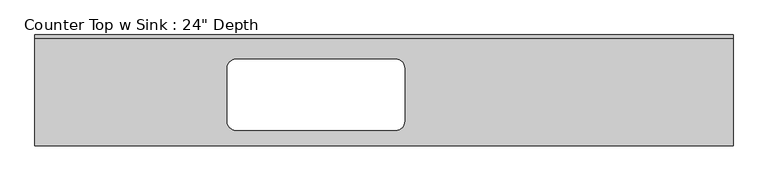
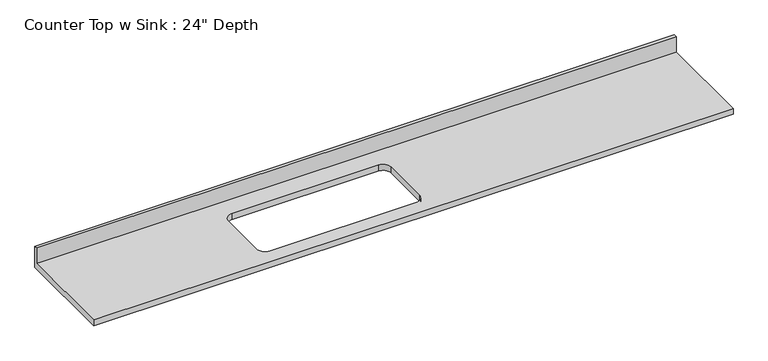
"""IFC4 building model written with IfcOpenShell, lengths in millimetres: furniture geometry."""

import ifcopenshell
import ifcopenshell.guid

model = None  # the IFC model being written
_history = None  # IfcOwnerHistory: only IFC2X3 demands one
_inside = {}  # id of a spatial element -> (the spatial element, [elements in it])
_under = {}  # id of a project, library or spatial element -> (it, [spatial elements below it])
_declared = {}  # id of a project -> (the project, [libraries it declares])
_typed = {}  # id of a type object -> (the type object, [elements of that type])
_made_of = {}  # id of a material, layer set ... -> (it, [elements and type objects made of it])


def new_model(schema):
    """Start an empty IFC model of exactly this schema.

    Asked for "IFC4X3", IfcOpenShell would pick the latest addendum, in which some entities
    have other attributes; the version numbers below select the first issue.
    IFC2X3 requires an IfcOwnerHistory on every rooted entity: one is made here for all.
    """
    global model, _history
    if schema == "IFC4X3":
        model = ifcopenshell.file(schema_version=(4, 3, 0, 0))
    else:
        model = ifcopenshell.file(schema=schema)
    _inside.clear()
    _under.clear()
    _declared.clear()
    _typed.clear()
    _made_of.clear()
    _history = None
    if model.schema == "IFC2X3":
        org = make("IfcOrganization", Name="unknown")
        user = make(
            "IfcPersonAndOrganization",
            ThePerson=make("IfcPerson", FamilyName="unknown"),
            TheOrganization=org,
        )
        app = make(
            "IfcApplication",
            ApplicationDeveloper=org,
            Version="unknown",
            ApplicationFullName="unknown",
            ApplicationIdentifier="unknown",
        )
        _history = make(
            "IfcOwnerHistory",
            OwningUser=user,
            OwningApplication=app,
            ChangeAction="ADDED",
            CreationDate=0,
        )
    return model


def make(cls, **values):
    """One entity of the class cls with the attributes given. An attribute that is None is left unset."""
    return model.create_entity(
        cls, **{name: value for name, value in values.items() if value is not None}
    )


def rooted(cls, **values):
    """An entity with a GlobalId (a new one), such as an element, a storey or a relation."""
    return make(cls, GlobalId=ifcopenshell.guid.new(), OwnerHistory=_history, **values)


def si_unit(unit_type, name, prefix=None):
    """IfcSIUnit, for example si_unit("LENGTHUNIT", "METRE", prefix="MILLI")."""
    return make("IfcSIUnit", UnitType=unit_type, Prefix=prefix, Name=name)


def assignment(units):
    """IfcUnitAssignment: the units of a project."""
    return None if units is None else make("IfcUnitAssignment", Units=units)


def point(xyz):
    """IfcCartesianPoint."""
    return None if xyz is None else make("IfcCartesianPoint", Coordinates=xyz)


def direction(xyz):
    """IfcDirection."""
    return None if xyz is None else make("IfcDirection", DirectionRatios=xyz)


def frame(location, z_axis=None, x_axis=None):
    """IfcAxis2Placement3D, a coordinate frame: its origin and axes. An axis left out is left unset."""
    return make(
        "IfcAxis2Placement3D",
        Location=point(location),
        Axis=direction(z_axis),
        RefDirection=direction(x_axis),
    )


def origin():
    """The frame at (0, 0, 0) with its axes left unset."""
    return frame((0.0, 0.0, 0.0))


def place(relative_to, where):
    """IfcLocalPlacement: puts the frame where relative to a parent placement (None: the world)."""
    return make(
        "IfcLocalPlacement", PlacementRelTo=relative_to, RelativePlacement=where
    )


def context(
    kind, dimensions, precision=None, world=None, true_north=None, identifier=None
):
    """IfcGeometricRepresentationContext, for example the 3D "Model" context."""
    return make(
        "IfcGeometricRepresentationContext",
        ContextIdentifier=identifier,
        ContextType=kind,
        CoordinateSpaceDimension=dimensions,
        Precision=precision,
        WorldCoordinateSystem=world,
        TrueNorth=true_north,
    )


def project(units=None, contexts=None):
    """IfcProject with its units and contexts."""
    return rooted(
        "IfcProject",
        Name="project",
        RepresentationContexts=contexts,
        UnitsInContext=assignment(units),
    )


def spatial(cls, under=None, at=None, **own):
    """A site, building, storey or space (cls), placed at a placement, below another one or the project."""
    s = rooted(cls, ObjectPlacement=at, **own)
    if under is not None:
        _under.setdefault(under.id(), (under, []))[1].append(s)
    return s


def polyline(points):
    """IfcPolyline through the points."""
    return make("IfcPolyline", Points=[point(p) for p in points])


def circle_curve(where, radius):
    """IfcCircle in the frame where."""
    return make("IfcCircle", Position=where, Radius=radius)


def shape(context_of_items, identifier, shape_type, items):
    """IfcShapeRepresentation: the items that make up one representation, for example the "Body"."""
    return make(
        "IfcShapeRepresentation",
        ContextOfItems=context_of_items,
        RepresentationIdentifier=identifier,
        RepresentationType=shape_type,
        Items=items,
    )


def source(mapping_origin, context_of_items, identifier, shape_type, items):
    """IfcRepresentationMap: a shape defined once, which mapped items show again and again."""
    return make(
        "IfcRepresentationMap",
        MappingOrigin=mapping_origin,
        MappedRepresentation=shape(context_of_items, identifier, shape_type, items),
    )


def transform(
    local_origin,
    x_axis=None,
    y_axis=None,
    z_axis=None,
    scale=None,
    scale2=None,
    scale3=None,
    uniform=True,
):
    """IfcCartesianTransformationOperator3D, or its non-uniform kind. x_axis, y_axis, z_axis: its Axis1, 2, 3."""
    if uniform:
        return make(
            "IfcCartesianTransformationOperator3D",
            Axis1=direction(x_axis),
            Axis2=direction(y_axis),
            LocalOrigin=point(local_origin),
            Scale=scale,
            Axis3=direction(z_axis),
        )
    return make(
        "IfcCartesianTransformationOperator3DnonUniform",
        Axis1=direction(x_axis),
        Axis2=direction(y_axis),
        LocalOrigin=point(local_origin),
        Scale=scale,
        Axis3=direction(z_axis),
        Scale2=scale2,
        Scale3=scale3,
    )


def mapped(mapping_source, mapping_target):
    """IfcMappedItem: shows the shape of a source again, moved by a transform."""
    return make(
        "IfcMappedItem", MappingSource=mapping_source, MappingTarget=mapping_target
    )


def made_of(thing, what):
    """Note that an element or type object is made of a material, layer set ...; save() writes the relation."""
    if what is not None:
        _made_of.setdefault(what.id(), (what, []))[1].append(thing)
    return thing


def element(
    cls,
    number,
    at=None,
    inside=None,
    cuts=None,
    type_object=None,
    material=None,
    context=None,
    identifier="Body",
    shape_type=None,
    held_by="IfcProductDefinitionShape",
    body=None,
    shapes=None,
    **own,
):
    """One element of the class cls, such as IfcWall. Its Tag is "e" and its number.

    at: its placement. inside: the storey or other place that contains it. cuts: it is an
    opening in that element (IfcRelVoidsElement). A single representation is given by context,
    identifier, shape_type and body (its items); several are given by shapes. held_by: the class
    of the entity that holds the representations. save() writes the other relations.
    """
    e = rooted(cls, Tag="e%d" % number, ObjectPlacement=at, **own)
    if body is not None:
        shapes = [shape(context, identifier, shape_type, body)]
    if shapes is not None:
        e.Representation = make(held_by, Representations=shapes)
    if inside is not None:
        _inside.setdefault(inside.id(), (inside, []))[1].append(e)
    if cuts is not None:
        rooted(
            "IfcRelVoidsElement", RelatingBuildingElement=cuts, RelatedOpeningElement=e
        )
    if type_object is not None:
        _typed.setdefault(type_object.id(), (type_object, []))[1].append(e)
    return made_of(e, material)


def aggregate(whole, parts):
    """IfcRelAggregates: a whole, such as a stair, and the parts it consists of."""
    return rooted("IfcRelAggregates", RelatingObject=whole, RelatedObjects=parts)


def save(model, path):
    """Write the relations noted so far, then the file.

    IfcRelAggregates (storeys below a building ...), IfcRelContainedInSpatialStructure (elements
    in a storey), IfcRelDefinesByType, IfcRelAssociatesMaterial and IfcRelDeclares: one each for
    every whole, place, type object, material and project.
    """
    for whole, parts in _under.values():
        aggregate(whole, parts)
    for where, things in _inside.values():
        rooted(
            "IfcRelContainedInSpatialStructure",
            RelatedElements=things,
            RelatingStructure=where,
        )
    for kind, things in _typed.values():
        rooted("IfcRelDefinesByType", RelatedObjects=things, RelatingType=kind)
    for what, things in _made_of.values():
        rooted("IfcRelAssociatesMaterial", RelatedObjects=things, RelatingMaterial=what)
    for by, libraries in _declared.values():
        rooted("IfcRelDeclares", RelatingContext=by, RelatedDefinitions=libraries)
    model.write(path)


def plane_surface(at):
    """IfcPlane: the flat surface through the origin of the frame at, square to its z axis."""
    return make("IfcPlane", Position=at)


def revolved_surface(curve, axis_point, axis_direction):
    """IfcSurfaceOfRevolution: the curve turned about the line through axis_point along axis_direction."""
    return make(
        "IfcSurfaceOfRevolution",
        SweptCurve=make("IfcArbitraryOpenProfileDef", ProfileType="CURVE", Curve=curve),
        AxisPosition=make("IfcAxis1Placement", Location=point(axis_point), Axis=direction(axis_direction)),
    )


def advanced_brep(points, edges, surfaces, faces):
    """IfcAdvancedBrep: a solid bounded by faces that lie on surfaces and meet in shared edges.

    An edge is (start, end): straight between two places in points (the first is 0);
    or (start, end, curve); or (start, end, curve, False) where it runs against its curve.
    A face is (place in surfaces, loops), or (place, loops, False) where it looks against
    its surface's normal. A loop lists edges by number (the first is 1), with a minus sign
    where the edge is run from its end to its start. The first loop is the outer one.
    """
    corners = [point(p) for p in points]
    vertices = [make("IfcVertexPoint", VertexGeometry=c) for c in corners]
    made = []
    for start, end, *more in edges:
        made.append(
            make(
                "IfcEdgeCurve",
                EdgeStart=vertices[start],
                EdgeEnd=vertices[end],
                EdgeGeometry=more[0] if more else make("IfcPolyline", Points=[corners[start], corners[end]]),
                SameSense=more[1] if len(more) > 1 else True,
            )
        )
    hull = []
    for where, loops, *sense in faces:
        bounds = []
        for j, loop in enumerate(loops):
            ring = [make("IfcOrientedEdge", EdgeElement=made[abs(k) - 1], Orientation=k > 0) for k in loop]
            bounds.append(
                make(
                    "IfcFaceOuterBound" if j == 0 else "IfcFaceBound",
                    Bound=make("IfcEdgeLoop", EdgeList=ring),
                    Orientation=True,
                )
            )
        hull.append(make("IfcAdvancedFace", Bounds=bounds, FaceSurface=surfaces[where], SameSense=sense[0] if sense else True))
    return make("IfcAdvancedBrep", Outer=make("IfcClosedShell", CfsFaces=hull))


def furniture_78cc09a6(model_context):
    return source(origin(), model_context, "Body", "AdvancedBrep", [
        advanced_brep(
        [(-1200.4622951, -635.0, 914.4), (2796.8627049, -635.0, 914.4), (2796.8627049, -19.05, 914.4), (-1200.4622951, -19.05, 914.4), (-48.9743878, -139.7, 914.4), (865.4256122, -139.7, 914.4), (916.2256122, -190.5, 914.4), (916.2256122, -495.3, 914.4), (865.4256122, -546.1, 914.4), (-48.9743878, -546.1, 914.4), (-99.7743878, -495.3, 914.4), (-99.7743878, -190.5, 914.4), (2796.8627049, 0.0, 876.3), (2796.8627049, -635.0, 876.3), (-1200.4622951, -635.0, 876.3), (-1200.4622951, 0.0, 876.3), (865.4256122, -139.7, 876.3), (-48.9743878, -139.7, 876.3), (-99.7743878, -190.5, 876.3), (-99.7743878, -495.3, 876.3), (-48.9743878, -546.1, 876.3), (865.4256122, -546.1, 876.3), (916.2256122, -495.3, 876.3), (916.2256122, -190.5, 876.3), (-1200.4622951, 0.0, 1016.0), (2796.8627049, 0.0, 1016.0), (-1200.4622951, -19.05, 1016.0), (2796.8627049, -19.05, 1016.0)],
        [
            (0, 1),
            (1, 2),
            (2, 3),
            (3, 0),
            (4, 5),
            (5, 6, circle_curve(frame((865.4256122, -190.5, 914.4), z_axis=(0.0, 0.0, -1.0), x_axis=(1.0, 0.0, 0.0)), 50.8)),
            (6, 7),
            (7, 8, circle_curve(frame((865.4256122, -495.3, 914.4), z_axis=(0.0, 0.0, -1.0), x_axis=(1.0, 0.0, 0.0)), 50.8)),
            (8, 9),
            (9, 10, circle_curve(frame((-48.9743878, -495.3, 914.4), z_axis=(0.0, 0.0, -1.0), x_axis=(1.0, 0.0, 0.0)), 50.8)),
            (10, 11),
            (11, 4, circle_curve(frame((-48.9743878, -190.5, 914.4), z_axis=(0.0, 0.0, -1.0), x_axis=(1.0, 0.0, 0.0)), 50.8)),
            (12, 13),
            (13, 14),
            (14, 15),
            (15, 12),
            (16, 17),
            (17, 18, circle_curve(frame((-48.9743878, -190.5, 876.3), z_axis=(0.0, 0.0, 1.0), x_axis=(1.0, 0.0, 0.0)), 50.8)),
            (18, 19),
            (19, 20, circle_curve(frame((-48.9743878, -495.3, 876.3), z_axis=(0.0, 0.0, 1.0), x_axis=(1.0, 0.0, 0.0)), 50.8)),
            (20, 21),
            (21, 22, circle_curve(frame((865.4256122, -495.3, 876.3), z_axis=(0.0, 0.0, 1.0), x_axis=(1.0, 0.0, 0.0)), 50.8)),
            (22, 23),
            (23, 16, circle_curve(frame((865.4256122, -190.5, 876.3), z_axis=(0.0, 0.0, 1.0), x_axis=(1.0, 0.0, 0.0)), 50.8)),
            (15, 24),
            (24, 25),
            (25, 12),
            (14, 0),
            (3, 26),
            (26, 24),
            (13, 1),
            (25, 27),
            (27, 2),
            (4, 17),
            (16, 5),
            (18, 11),
            (10, 19),
            (20, 9),
            (8, 21),
            (22, 7),
            (6, 23),
            (26, 27),
        ],
        [
            plane_surface(frame((-1200.4622951, 0.0, 914.4), z_axis=(0.0, 0.0, 1.0), x_axis=(-1.0, 0.0, 0.0))),
            plane_surface(frame((-1200.4622951, 0.0, 876.3), z_axis=(0.0, 0.0, -1.0), x_axis=(1.0, 0.0, 0.0))),
            plane_surface(frame((2796.8627049, 0.0, 914.4), z_axis=(0.0, 1.0, 0.0), x_axis=(0.0, 0.0, -1.0))),
            plane_surface(frame((-1200.4622951, 0.0, 914.4), z_axis=(-1.0, 0.0, 0.0), x_axis=(0.0, 0.0, -1.0))),
            plane_surface(frame((-1200.4622951, -635.0, 914.4), z_axis=(0.0, -1.0, 0.0), x_axis=(0.0, 0.0, -1.0))),
            plane_surface(frame((2796.8627049, -635.0, 914.4), z_axis=(1.0, 0.0, 0.0), x_axis=(0.0, 0.0, -1.0))),
            plane_surface(frame((865.4256122, -139.7, 914.4), z_axis=(0.0, -1.0, 0.0), x_axis=(0.0, 0.0, -1.0))),
            plane_surface(frame((-99.7743878, -190.5, 914.4), z_axis=(1.0, 0.0, 0.0), x_axis=(0.0, 0.0, -1.0))),
            plane_surface(frame((-48.9743878, -546.1, 914.4), z_axis=(0.0, 1.0, 0.0), x_axis=(0.0, 0.0, -1.0))),
            plane_surface(frame((916.2256122, -495.3, 914.4), z_axis=(-1.0, 0.0, 0.0), x_axis=(0.0, 0.0, -1.0))),
            revolved_surface(polyline([(1.8256121999999948, -190.5, 914.4), (1.8256121999999948, -190.5, 876.3)]), (-48.9743878, -190.5, 876.3), (0.0, 0.0, 1.0)),
            revolved_surface(polyline([(916.2256122, -495.3, 914.4), (916.2256122, -495.3, 876.3)]), (865.4256122, -495.3, 876.3), (0.0, 0.0, 1.0)),
            revolved_surface(polyline([(916.2256122, -190.5, 914.4), (916.2256122, -190.5, 876.3)]), (865.4256122, -190.5, 876.3), (0.0, 0.0, 1.0)),
            revolved_surface(polyline([(1.8256121999999948, -495.3, 914.4), (1.8256121999999948, -495.3, 876.3)]), (-48.9743878, -495.3, 876.3), (0.0, 0.0, 1.0)),
            plane_surface(frame((-1200.4622951, 0.0, 1016.0), z_axis=(0.0, 0.0, 1.0), x_axis=(0.0, -1.0, 0.0))),
            plane_surface(frame((-1200.4622951, -19.05, 1016.0), z_axis=(0.0, -1.0, 0.0), x_axis=(0.0, 0.0, -1.0))),
        ],
        [
            (0, [[1, 2, 3, 4], [5, 6, 7, 8, 9, 10, 11, 12]]),
            (1, [[13, 14, 15, 16], [17, 18, 19, 20, 21, 22, 23, 24]]),
            (2, [[-16, 25, 26, 27]]),
            (3, [[-15, 28, -4, 29, 30, -25]]),
            (4, [[-1, -28, -14, 31]]),
            (5, [[-13, -27, 32, 33, -2, -31]]),
            (6, [[34, -17, 35, -5]]),
            (7, [[36, -11, 37, -19]]),
            (8, [[38, -9, 39, -21]]),
            (9, [[40, -7, 41, -23]]),
            (10, [[-34, -12, -36, -18]]),
            (11, [[-39, -8, -40, -22]]),
            (12, [[-35, -24, -41, -6]]),
            (13, [[-37, -10, -38, -20]]),
            (14, [[-30, 42, -32, -26]]),
            (15, [[-42, -29, -3, -33]]),
        ],
    ),
    ])


if __name__ == "__main__":
    model = new_model("IFC4")
    model_context = context("Model", 3, world=origin())
    ifc_project = project(units=[si_unit("LENGTHUNIT", "METRE", prefix="MILLI")], contexts=[model_context])
    site = spatial("IfcSite", under=ifc_project)
    building = spatial("IfcBuilding", under=site)
    placement = place(None, origin())
    furniture_shape = furniture_78cc09a6(model_context)
    element("IfcFurniture", 1, ObjectType="Counter Top w Sink : 24\" Depth", at=placement, inside=building, context=model_context, shape_type="MappedRepresentation", body=[
        mapped(furniture_shape, transform((0.0, 0.0, 0.0), x_axis=(1.0, 0.0, 0.0), y_axis=(0.0, 1.0, 0.0), z_axis=(0.0, 0.0, 1.0))),
    ])
    save(model, "model.ifc")

# Revit data of these elements
# Type "Counter Top w Sink : 24\" Depth"
#   Assembly Code = "C1030400"
#   Counter Thickness = 0' - 1 1/2"
#   Depth = 2' - 1"
#   Height = 3' - 0"
#   Length [instance default] = 8' - 0"
#   Sink Location [instance default] = 2' - 0"
#   Sink Location To Wall [instance default] = 0' - 6"
#   Sink Opening Depth [instance default] = 1' - 3"
#   Sink Opening Width [instance default] = 3' - 3"
#   Counter Top Material = none
#   Default Elevation = 0
# Element 1 (IfcFurniture, "Counter Top w Sink : 24\" Depth")
#   Length = 13' - 1 3/8"
#   Sink Location = 5' - 3.33417"
#   Materials on its faces: "Counter Top"
# Materials
#   "Counter Top": class "Wood", colour RGB 226 177 128, transparency 0
